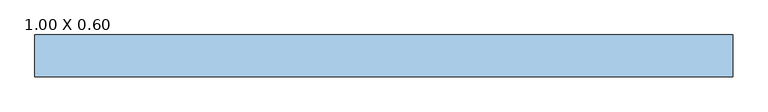
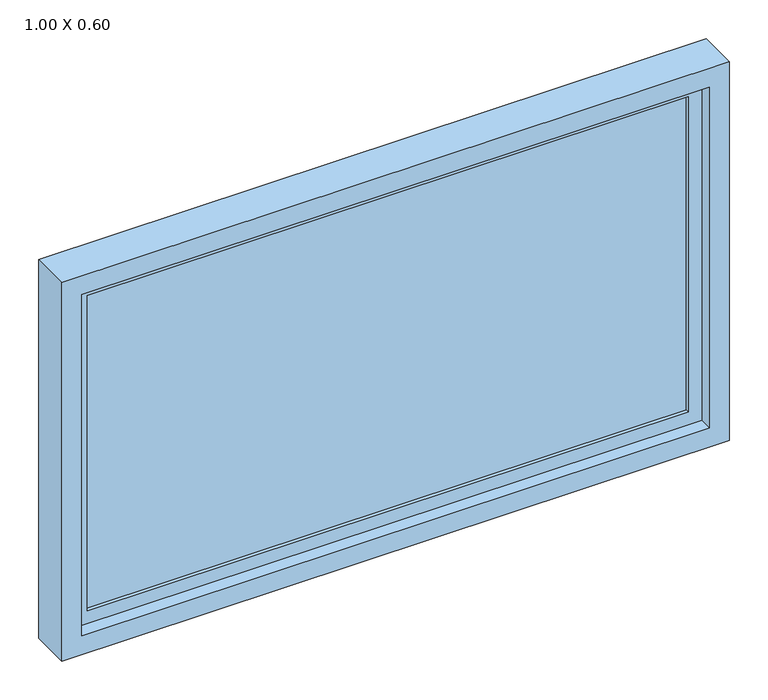
"""IFC4 building model written with IfcOpenShell, lengths in millimetres: window geometry, .CC_ND 300_MAXIM-AR : 1.00 X 0.60."""

import ifcopenshell
import ifcopenshell.guid

model = None  # the IFC model being written
_history = None  # IfcOwnerHistory: only IFC2X3 demands one
_inside = {}  # id of a spatial element -> (the spatial element, [elements in it])
_under = {}  # id of a project, library or spatial element -> (it, [spatial elements below it])
_declared = {}  # id of a project -> (the project, [libraries it declares])
_typed = {}  # id of a type object -> (the type object, [elements of that type])
_made_of = {}  # id of a material, layer set ... -> (it, [elements and type objects made of it])


def new_model(schema):
    """Start an empty IFC model of exactly this schema.

    Asked for "IFC4X3", IfcOpenShell would pick the latest addendum, in which some entities
    have other attributes; the version numbers below select the first issue.
    IFC2X3 requires an IfcOwnerHistory on every rooted entity: one is made here for all.
    """
    global model, _history
    if schema == "IFC4X3":
        model = ifcopenshell.file(schema_version=(4, 3, 0, 0))
    else:
        model = ifcopenshell.file(schema=schema)
    _inside.clear()
    _under.clear()
    _declared.clear()
    _typed.clear()
    _made_of.clear()
    _history = None
    if model.schema == "IFC2X3":
        org = make("IfcOrganization", Name="unknown")
        user = make(
            "IfcPersonAndOrganization",
            ThePerson=make("IfcPerson", FamilyName="unknown"),
            TheOrganization=org,
        )
        app = make(
            "IfcApplication",
            ApplicationDeveloper=org,
            Version="unknown",
            ApplicationFullName="unknown",
            ApplicationIdentifier="unknown",
        )
        _history = make(
            "IfcOwnerHistory",
            OwningUser=user,
            OwningApplication=app,
            ChangeAction="ADDED",
            CreationDate=0,
        )
    return model


def make(cls, **values):
    """One entity of the class cls with the attributes given. An attribute that is None is left unset."""
    return model.create_entity(
        cls, **{name: value for name, value in values.items() if value is not None}
    )


def rooted(cls, **values):
    """An entity with a GlobalId (a new one), such as an element, a storey or a relation."""
    return make(cls, GlobalId=ifcopenshell.guid.new(), OwnerHistory=_history, **values)


def si_unit(unit_type, name, prefix=None):
    """IfcSIUnit, for example si_unit("LENGTHUNIT", "METRE", prefix="MILLI")."""
    return make("IfcSIUnit", UnitType=unit_type, Prefix=prefix, Name=name)


def assignment(units):
    """IfcUnitAssignment: the units of a project."""
    return None if units is None else make("IfcUnitAssignment", Units=units)


def point(xyz):
    """IfcCartesianPoint."""
    return None if xyz is None else make("IfcCartesianPoint", Coordinates=xyz)


def direction(xyz):
    """IfcDirection."""
    return None if xyz is None else make("IfcDirection", DirectionRatios=xyz)


def frame(location, z_axis=None, x_axis=None):
    """IfcAxis2Placement3D, a coordinate frame: its origin and axes. An axis left out is left unset."""
    return make(
        "IfcAxis2Placement3D",
        Location=point(location),
        Axis=direction(z_axis),
        RefDirection=direction(x_axis),
    )


def origin():
    """The frame at (0, 0, 0) with its axes left unset."""
    return frame((0.0, 0.0, 0.0))


def place(relative_to, where):
    """IfcLocalPlacement: puts the frame where relative to a parent placement (None: the world)."""
    return make(
        "IfcLocalPlacement", PlacementRelTo=relative_to, RelativePlacement=where
    )


def context(
    kind, dimensions, precision=None, world=None, true_north=None, identifier=None
):
    """IfcGeometricRepresentationContext, for example the 3D "Model" context."""
    return make(
        "IfcGeometricRepresentationContext",
        ContextIdentifier=identifier,
        ContextType=kind,
        CoordinateSpaceDimension=dimensions,
        Precision=precision,
        WorldCoordinateSystem=world,
        TrueNorth=true_north,
    )


def project(units=None, contexts=None):
    """IfcProject with its units and contexts."""
    return rooted(
        "IfcProject",
        Name="project",
        RepresentationContexts=contexts,
        UnitsInContext=assignment(units),
    )


def spatial(cls, under=None, at=None, **own):
    """A site, building, storey or space (cls), placed at a placement, below another one or the project."""
    s = rooted(cls, ObjectPlacement=at, **own)
    if under is not None:
        _under.setdefault(under.id(), (under, []))[1].append(s)
    return s


def polyline(points):
    """IfcPolyline through the points."""
    return make("IfcPolyline", Points=[point(p) for p in points])


def outline(outer, holes=None, kind="AREA"):
    """IfcArbitraryClosedProfileDef: a profile drawn as a closed curve; with holes, ...WithVoids."""
    if holes is None:
        return make("IfcArbitraryClosedProfileDef", ProfileType=kind, OuterCurve=outer)
    return make(
        "IfcArbitraryProfileDefWithVoids",
        ProfileType=kind,
        OuterCurve=outer,
        InnerCurves=holes,
    )


def extrude(swept, where, along, depth):
    """IfcExtrudedAreaSolid: the profile swept, set in the frame where, extruded along a direction by depth."""
    return make(
        "IfcExtrudedAreaSolid",
        SweptArea=swept,
        Position=where,
        ExtrudedDirection=direction(along),
        Depth=depth,
    )


def shape(context_of_items, identifier, shape_type, items):
    """IfcShapeRepresentation: the items that make up one representation, for example the "Body"."""
    return make(
        "IfcShapeRepresentation",
        ContextOfItems=context_of_items,
        RepresentationIdentifier=identifier,
        RepresentationType=shape_type,
        Items=items,
    )


def source(mapping_origin, context_of_items, identifier, shape_type, items):
    """IfcRepresentationMap: a shape defined once, which mapped items show again and again."""
    return make(
        "IfcRepresentationMap",
        MappingOrigin=mapping_origin,
        MappedRepresentation=shape(context_of_items, identifier, shape_type, items),
    )


def transform(
    local_origin,
    x_axis=None,
    y_axis=None,
    z_axis=None,
    scale=None,
    scale2=None,
    scale3=None,
    uniform=True,
):
    """IfcCartesianTransformationOperator3D, or its non-uniform kind. x_axis, y_axis, z_axis: its Axis1, 2, 3."""
    if uniform:
        return make(
            "IfcCartesianTransformationOperator3D",
            Axis1=direction(x_axis),
            Axis2=direction(y_axis),
            LocalOrigin=point(local_origin),
            Scale=scale,
            Axis3=direction(z_axis),
        )
    return make(
        "IfcCartesianTransformationOperator3DnonUniform",
        Axis1=direction(x_axis),
        Axis2=direction(y_axis),
        LocalOrigin=point(local_origin),
        Scale=scale,
        Axis3=direction(z_axis),
        Scale2=scale2,
        Scale3=scale3,
    )


def mapped(mapping_source, mapping_target):
    """IfcMappedItem: shows the shape of a source again, moved by a transform."""
    return make(
        "IfcMappedItem", MappingSource=mapping_source, MappingTarget=mapping_target
    )


def made_of(thing, what):
    """Note that an element or type object is made of a material, layer set ...; save() writes the relation."""
    if what is not None:
        _made_of.setdefault(what.id(), (what, []))[1].append(thing)
    return thing


def element(
    cls,
    number,
    at=None,
    inside=None,
    cuts=None,
    type_object=None,
    material=None,
    context=None,
    identifier="Body",
    shape_type=None,
    held_by="IfcProductDefinitionShape",
    body=None,
    shapes=None,
    **own,
):
    """One element of the class cls, such as IfcWall. Its Tag is "e" and its number.

    at: its placement. inside: the storey or other place that contains it. cuts: it is an
    opening in that element (IfcRelVoidsElement). A single representation is given by context,
    identifier, shape_type and body (its items); several are given by shapes. held_by: the class
    of the entity that holds the representations. save() writes the other relations.
    """
    e = rooted(cls, Tag="e%d" % number, ObjectPlacement=at, **own)
    if body is not None:
        shapes = [shape(context, identifier, shape_type, body)]
    if shapes is not None:
        e.Representation = make(held_by, Representations=shapes)
    if inside is not None:
        _inside.setdefault(inside.id(), (inside, []))[1].append(e)
    if cuts is not None:
        rooted(
            "IfcRelVoidsElement", RelatingBuildingElement=cuts, RelatedOpeningElement=e
        )
    if type_object is not None:
        _typed.setdefault(type_object.id(), (type_object, []))[1].append(e)
    return made_of(e, material)


def aggregate(whole, parts):
    """IfcRelAggregates: a whole, such as a stair, and the parts it consists of."""
    return rooted("IfcRelAggregates", RelatingObject=whole, RelatedObjects=parts)


def save(model, path):
    """Write the relations noted so far, then the file.

    IfcRelAggregates (storeys below a building ...), IfcRelContainedInSpatialStructure (elements
    in a storey), IfcRelDefinesByType, IfcRelAssociatesMaterial and IfcRelDeclares: one each for
    every whole, place, type object, material and project.
    """
    for whole, parts in _under.values():
        aggregate(whole, parts)
    for where, things in _inside.values():
        rooted(
            "IfcRelContainedInSpatialStructure",
            RelatedElements=things,
            RelatingStructure=where,
        )
    for kind, things in _typed.values():
        rooted("IfcRelDefinesByType", RelatedObjects=things, RelatingType=kind)
    for what, things in _made_of.values():
        rooted("IfcRelAssociatesMaterial", RelatedObjects=things, RelatingMaterial=what)
    for by, libraries in _declared.values():
        rooted("IfcRelDeclares", RelatingContext=by, RelatedDefinitions=libraries)
    model.write(path)


def window_1_00_x_0_60_b9f016d9(model_context):
    return source(origin(), model_context, "Body", "SweptSolid", [
        extrude(outline(polyline([(-450.0, -4.0), (-450.0, 4.0), (450.0, 4.0), (450.0, -4.0), (-450.0, -4.0)])), frame((0.0, 0.0, 1550.0), z_axis=(0.0, 0.0, 1.0), x_axis=(1.0, 0.0, 0.0)), (0.0, 0.0, 1.0), 500.0),
        extrude(outline(polyline([(1530.0, 470.0), (2070.0, 470.0), (2070.0, -470.0), (1530.0, -470.0), (1530.0, 470.0)]), holes=[polyline([(2050.0, 450.0), (1550.0, 450.0), (1550.0, -450.0), (2050.0, -450.0), (2050.0, 450.0)])]), frame((0.0, -10.0, 0.0), z_axis=(0.0, 1.0, 0.0), x_axis=(0.0, 0.0, 1.0)), (0.0, 0.0, 1.0), 20.0),
        extrude(outline(polyline([(1500.0, 500.0), (2100.0, 500.0), (2100.0, -500.0), (1500.0, -500.0), (1500.0, 500.0)]), holes=[polyline([(2070.0, 470.0), (1530.0, 470.0), (1530.0, -470.0), (2070.0, -470.0), (2070.0, 470.0)])]), frame((0.0, -30.0, 0.0), z_axis=(0.0, 1.0, 0.0), x_axis=(0.0, 0.0, 1.0)), (0.0, 0.0, 1.0), 60.0),
    ])


if __name__ == "__main__":
    model = new_model("IFC4")
    model_context = context("Model", 3, world=origin())
    ifc_project = project(units=[si_unit("LENGTHUNIT", "METRE", prefix="MILLI")], contexts=[model_context])
    site = spatial("IfcSite", under=ifc_project)
    building = spatial("IfcBuilding", under=site)
    placement = place(None, origin())
    window_1_00_x_0_60_shape = window_1_00_x_0_60_b9f016d9(model_context)
    element("IfcWindow", 1, ObjectType=".CC_ND 300_MAXIM-AR : 1.00 X 0.60", at=placement, inside=building, context=model_context, shape_type="MappedRepresentation", body=[
        mapped(window_1_00_x_0_60_shape, transform((0.0, 0.0, 0.0), x_axis=(1.0, 0.0, 0.0), y_axis=(0.0, 1.0, 0.0), z_axis=(0.0, 0.0, 1.0))),
    ])
    save(model, "model.ifc")

# Revit data of these elements
# Type ".CC_ND 300_MAXIM-AR : 1.00 X 0.60"
#   Type Mark = "67"
#   Largura Painel [instance default] = 0.02 m
#   Largura Esquadria [instance default] = 0.06 m
#   Espessura Vidro [instance default] = 0.008 m
#   Espessura Painel [instance default] = 0.02 m
#   Espessura Esquadria [instance default] = 0.03 m
#   Height = 0.60 m
#   Altura-padrão do peitoril = 1.50 m
#   Width = 1.00 m
#   Vidro = .VIDRO GENÉRICO
#   Esquadria = .ALUMÍNIO COM PINTURA ELETROSTÁTICA BRANCA
#   Wall Closure = (empty or 0)
# Element 1 (IfcWindow, ".CC_ND 300_MAXIM-AR : 1.00 X 0.60")
#   Materials on its faces: ".ALUMÍNIO COM PINTURA ELETROSTÁTICA BRANCA", ".VIDRO GENÉRICO"
# Materials
#   ".VIDRO GENÉRICO": class ".CC_VIDRO", colour RGB 0 128 192, transparency 0.9, Description = "Vidro comum", Cost = 0
#   ".ALUMÍNIO COM PINTURA ELETROSTÁTICA BRANCA": class "CC_METAIS", colour RGB 241 241 241, transparency 0, Cost = 0
